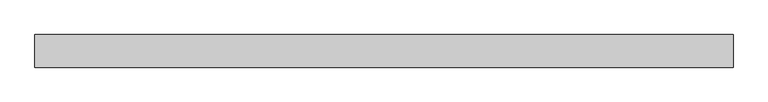
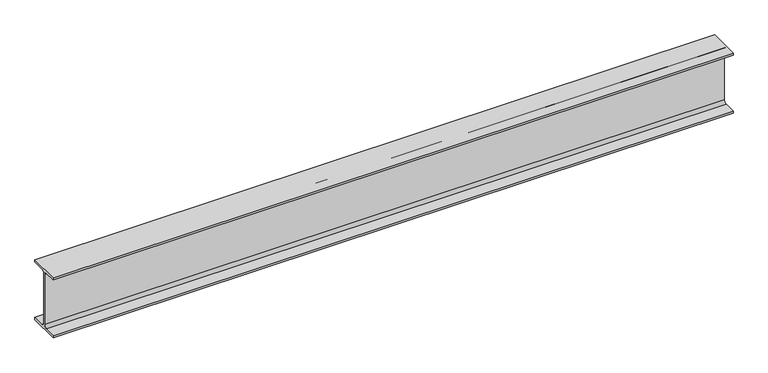
"""IFC4 building model written with IfcOpenShell, lengths in millimetres: beam geometry, 0912_Steel Framing_H-KSD3502 : H_SB_ASB_H-250x125x6x9."""

from ifc_helpers import new_model, si_unit, point, frame, frame_2d, origin, place, context, project, spatial, polyline, circle_curve, trimmed, segment, composite_curve, outline, extrude, source, transform, mapped, element, save


def beam_8759ffc8(model_context):
    return source(origin(), model_context, "Body", "SweptSolid", [
        extrude(outline(composite_curve([segment(polyline([(62.5, -116.0), (62.5, -125.0), (-62.5, -125.0), (-62.5, -116.0), (-15.0, -116.0)]), True, "CONTINUOUS"), segment(trimmed(circle_curve(frame_2d((-15.0, -104.0)), 12.0), [point((-15.0, -116.0))], [point((-3.0, -104.0))], True, "CARTESIAN"), True, "CONTINUOUS"), segment(polyline([(-3.0, -104.0), (-3.0, 104.0)]), True, "CONTINUOUS"), segment(trimmed(circle_curve(frame_2d((-15.0, 104.0)), 12.0), [point((-3.0, 104.0))], [point((-15.0, 116.0))], True, "CARTESIAN"), True, "CONTINUOUS"), segment(polyline([(-15.0, 116.0), (-62.5, 116.0), (-62.5, 125.0), (62.5, 125.0), (62.5, 116.0), (15.0, 116.0)]), True, "CONTINUOUS"), segment(trimmed(circle_curve(frame_2d((15.0, 104.0)), 12.0), [point((15.0, 116.0))], [point((3.0, 104.0))], True, "CARTESIAN"), True, "CONTINUOUS"), segment(polyline([(3.0, 104.0), (3.0, -104.0)]), True, "CONTINUOUS"), segment(trimmed(circle_curve(frame_2d((15.0, -104.0)), 12.0), [point((3.0, -104.0))], [point((15.0, -116.0))], True, "CARTESIAN"), True, "CONTINUOUS"), segment(polyline([(15.0, -116.0), (62.5, -116.0)]), True, "CONTINUOUS")], self_intersect=False)), frame((-1337.3, 0.0, 0.0), z_axis=(1.0, 0.0, 0.0), x_axis=(0.0, 1.0, 0.0)), (0.0, 0.0, 1.0), 2674.6),
    ])


if __name__ == "__main__":
    model = new_model("IFC4")
    model_context = context("Model", 3, world=origin())
    ifc_project = project(units=[si_unit("LENGTHUNIT", "METRE", prefix="MILLI")], contexts=[model_context])
    site = spatial("IfcSite", under=ifc_project)
    building = spatial("IfcBuilding", under=site)
    placement = place(None, origin())
    beam_shape = beam_8759ffc8(model_context)
    element("IfcBeam", 1, ObjectType="0912_Steel Framing_H-KSD3502 : H_SB_ASB_H-250x125x6x9", at=placement, inside=building, context=model_context, shape_type="MappedRepresentation", body=[
        mapped(beam_shape, transform((0.0, 0.0, 0.0), x_axis=(1.0, 0.0, 0.0), y_axis=(0.0, 1.0, 0.0), z_axis=(0.0, 0.0, 1.0))),
    ])
    save(model, "model.ifc")

# Revit data of these elements
# Type "0912_Steel Framing_H-KSD3502 : H_SB_ASB_H-250x125x6x9"
#   H_WM Code_1 = "S01AA003-00001 | Main Steel Structure Fabrication Work | Shelter/Building | Light Steel - Standard (30KG/M>Weight) | Material: (   )"
#   H_WM Code_2 = "S03AA029-00001 | Main Steel Structure Erection Work | Shelter/Building | Light Steel (30KG/M>Weight) | Material: (   )"
#   H_WM Code_3 = "S01AA010-00001 | Main Steel Structure Fabrication Work | Shelter/Building | Steel Painting/Coating | for Non-Fireproofed Steel Surface, Surface Preparation, Primer, Second & Final Coat | Material: (   )"
#   H_Q'ty Cal Type Tag = "SB-Q2"
#   Width = 12.5 cm
#   Web Thickness = 0.6 cm
#   Web Fillet = 1.2 cm
#   Warping Constant = 42539.8 cm⁶
#   W = 0
#   Torsional Moment of Inertia = 7.8102 cm⁴
#   Section Area = 37.66 cm²
#   Plastic Modulus weak axis = 73.1 cm³
#   Plastic Modulus strong axis = 366.0 cm³
#   Perimeter = 0.97 m²/m
#   Nominal Weight = 29.60 kgf/m
#   Moment of Inertia weak axis = 294.00 cm⁴
#   Moment of Inertia strong axis = 4050.00 cm⁴
#   Height = 25.0 cm
#   Flange Thickness = 0.9 cm
#   Elastic Modulus weak axis = 47.0 cm³
#   Elastic Modulus strong axis = 324.0 cm³
#   Centroid Vertical = 12.5 cm
#   Centroid Horizontal = 6.25 cm
#   Ix = 40500000
#   Length [instance default] = 1.5240 m
#   Zx = 366000
#   b = 0.1250 m
#   h = 0.2500 m
#   r = 0.0120 m
#   s = 0.0060 m
#   t = 0.0090 m
#   A = 0.003766 m²
#   Structural Material [instance default] = Steel, 45-345
#   Assembly Code = ""
# Element 1 (IfcBeam, "0912_Steel Framing_H-KSD3502 : H_SB_ASB_H-250x125x6x9")
#   Structural Material = none
# Materials
#   "Steel, 45-345": class "Metal", colour RGB 189 187 185, transparency 0, Description = "Steel 345 MPa", Cost = 0
